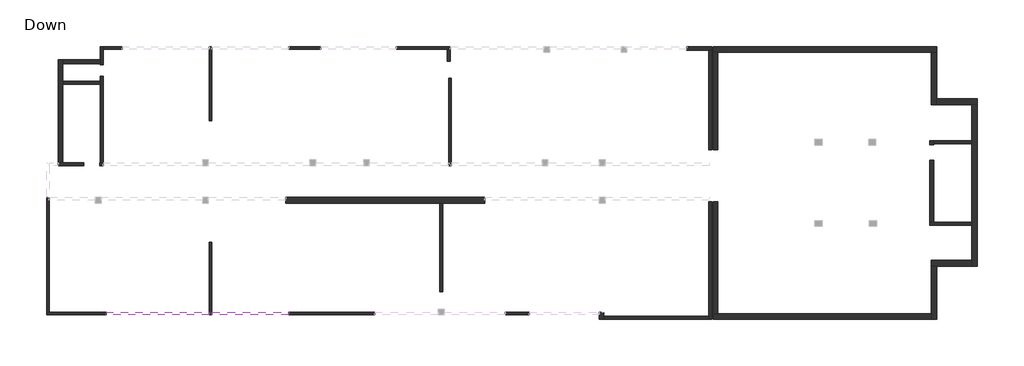
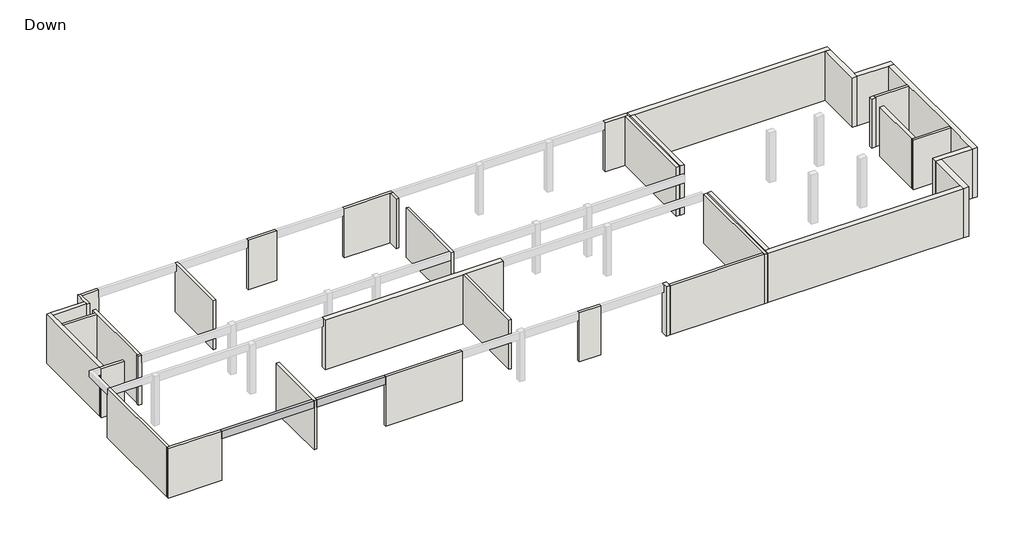
# One storey, part 1 of 2: 38 walls, 2 beams.
"""IFC4 building model written with IfcOpenShell, lengths in millimetres."""

from ifc_helpers import new_model, si_unit, origin, origin_with_axes, place, context, project, spatial, polyline, outline, extrude, faceted_brep, element, save

model = new_model("IFC4")

# Units and contexts
model_context = context("Model", 3, world=origin())
ifc_project = project(units=[si_unit("LENGTHUNIT", "METRE", prefix="MILLI")], contexts=[model_context])

# Site, building, storey
site = spatial("IfcSite", under=ifc_project)
building = spatial("IfcBuilding", under=site)
storey = spatial("IfcBuildingStorey", under=building, Name="Down", Elevation=0.0)

# Beams
placement = place(None, origin())
element("IfcBeam", 1, ObjectType="Concrete Rectengular Beam : 20/65", at=placement, inside=storey, context=model_context, shape_type="Brep", body=[
    faceted_brep([(-12691.9389092, -4274.5314528, 4000.0), (-12691.9389092, -4074.5314528, 4000.0), (-19792.231636, -4074.5314528, 4000.0), (-19792.231636, -4274.5314528, 4000.0), (-12691.9389092, -4274.5314528, 3400.0), (-19792.231636, -4274.5314528, 3400.0), (-12691.9389092, -4074.5314528, 3400.0), (-19792.231636, -4074.5314528, 3400.0), (-19792.231636, -4074.5314528, 3730.0), (-12691.9389092, -4074.5314528, 3730.0)], [[[0, 1, 2, 3]], [[4, 0, 3, 5]], [[6, 4, 5, 7]], [[6, 7, 8, 2, 1, 9]], [[0, 4, 6, 9, 1]], [[5, 3, 2, 8, 7]]]),
])
element("IfcBeam", 2, ObjectType="Concrete Rectengular Beam : 20/65", at=placement, inside=storey, context=model_context, shape_type="Brep", body=[
    faceted_brep([(-12491.9389092, -4074.5314528, 4000.0), (-12491.9389092, -4274.5314528, 4000.0), (-7191.8713568, -4274.5314528, 4000.0), (-7191.8713568, -4074.5314528, 4000.0), (-12491.9389092, -4274.5314528, 3400.0), (-7191.8713568, -4274.5314528, 3400.0), (-12491.9389092, -4074.5314528, 3400.0), (-7191.8713568, -4074.5314528, 3400.0), (-12491.9389092, -4074.5314528, 3730.0), (-7191.8713568, -4074.5314528, 3730.0)], [[[0, 1, 2, 3]], [[1, 4, 5, 2]], [[4, 6, 7, 5]], [[7, 6, 8, 0, 3, 9]], [[4, 1, 0, 8, 6]], [[2, 5, 7, 9, 3]]]),
])

# Walls
element("IfcWall", 3, ObjectType="20", at=placement, inside=storey, context=model_context, shape_type="Brep", body=[
    faceted_brep([(-19792.231636, -4074.5314528, 0.0), (-23692.1640837, -4074.5314528, 0.0), (-23892.1640837, -4074.5314528, 0.0), (-23892.1640837, -4074.5314528, 4000.0), (-23692.1640837, -4074.5314528, 4000.0), (-19792.231636, -4074.5314528, 4000.0), (-19792.231636, -4074.5314528, 3400.0), (-19792.231636, -4274.5314528, 0.0), (-19792.231636, -4274.5314528, 3400.0), (-19792.231636, -4274.5314528, 4000.0), (-23892.1640837, -4274.5314528, 4000.0), (-23892.1640837, -4274.5314528, 0.0)], [[[0, 1, 2, 3, 4, 5, 6]], [[7, 8, 9, 10, 11]], [[2, 1, 0, 7, 11]], [[5, 4, 3, 10, 9]], [[0, 6, 5, 9, 8, 7]], [[3, 2, 11, 10]]]),
])
element("IfcWall", 4, ObjectType="20", at=placement, inside=storey, context=model_context, shape_type="Brep", body=[
    faceted_brep([(-23692.1640837, -4074.5314528, 0.0), (-23692.1640837, 3825.8513439, 0.0), (-23692.1640837, 3825.8513439, 3500.0), (-23692.1640837, 3825.8513439, 4000.0), (-23692.1640837, 3625.8513439, 4000.0), (-23692.1640837, -4074.5314528, 4000.0), (-23692.1640837, -4074.5314528, 3730.0), (-23892.1640837, -4074.5314528, 0.0), (-23892.1640837, -4074.5314528, 4000.0), (-23892.1640837, 3825.8513439, 4000.0), (-23892.1640837, 3825.8513439, 3500.0), (-23892.1640837, 3825.8513439, 0.0)], [[[0, 1, 2, 3, 4, 5, 6]], [[7, 8, 9, 10, 11]], [[1, 0, 7, 11]], [[3, 2, 1, 11, 10, 9]], [[5, 4, 3, 9, 8]], [[0, 6, 5, 8, 7]]]),
])
element("IfcWall", 5, ObjectType="20", at=placement, inside=storey, context=model_context, shape_type="Brep", body=[
    faceted_brep([(-23092.0740139, 6025.0407157, 0.0), (-21341.6124061, 6025.0407157, 0.0), (-21341.6124061, 6025.0407157, 4000.0), (-23092.0740139, 6025.0407157, 4000.0), (-23092.0740139, 6025.0407157, 3500.0), (-23092.0740139, 6225.0407157, 0.0), (-23092.0740139, 6225.0407157, 3500.0), (-23092.0740139, 6225.0407157, 4000.0), (-22792.0740139, 6225.0407157, 4000.0), (-21341.6124061, 6225.0407157, 4000.0), (-21341.6124061, 6225.0407157, 0.0), (-22792.0740139, 6225.0407157, 0.0)], [[[0, 1, 2, 3, 4]], [[5, 6, 7, 8, 9, 10, 11]], [[1, 0, 5, 11, 10]], [[2, 1, 10, 9]], [[3, 2, 9, 8, 7]], [[0, 4, 3, 7, 6, 5]]]),
])
element("IfcWall", 6, ObjectType="20", at=placement, inside=storey, context=model_context, shape_type="Brep", body=[
    faceted_brep([(-20240.9594, 6025.0407157, 0.0), (-19991.1958333, 6025.0407157, 0.0), (-19991.1958333, 6025.0407157, 3400.0), (-19991.1958333, 6025.0407157, 4000.0), (-20240.9594, 6025.0407157, 4000.0), (-20240.9594, 6225.0407157, 0.0), (-20240.9594, 6225.0407157, 4000.0), (-20191.1958333, 6225.0407157, 4000.0), (-19991.1958333, 6225.0407157, 4000.0), (-19991.1958333, 6225.0407157, 3400.0), (-19991.1958333, 6225.0407157, 0.0), (-20191.1958333, 6225.0407157, 0.0)], [[[0, 1, 2, 3, 4]], [[5, 6, 7, 8, 9, 10, 11]], [[1, 0, 5, 11, 10]], [[4, 3, 8, 7, 6]], [[0, 4, 6, 5]], [[3, 2, 1, 10, 9, 8]]]),
])
element("IfcWall", 7, ObjectType="20", at=placement, inside=storey, context=model_context, shape_type="Brep", body=[
    faceted_brep([(-19991.1958333, 6225.0407157, 0.0), (-19991.1958333, 12173.8810669, 0.0), (-19991.1958333, 12173.8810669, 4000.0), (-19991.1958333, 6225.0407157, 4000.0), (-19991.1958333, 6225.0407157, 3730.0), (-20191.1958333, 6225.0407157, 0.0), (-20191.1958333, 6225.0407157, 4000.0), (-20191.1958333, 12173.8810669, 4000.0), (-20191.1958333, 12173.8810669, 0.0)], [[[0, 1, 2, 3, 4]], [[5, 6, 7, 8]], [[1, 0, 5, 8]], [[2, 1, 8, 7]], [[3, 2, 7, 6]], [[0, 4, 3, 6, 5]]]),
])
element("IfcWall", 8, ObjectType="20", at=placement, inside=storey, context=model_context, shape_type="SweptSolid", body=[
    extrude(outline(polyline([(-22792.0740139, 11825.6712043), (-20192.2766709, 11825.6712043), (-20192.2766709, 11625.6712043), (-22792.0740139, 11625.6712043), (-22792.0740139, 11825.6712043)])), origin_with_axes(), (0.0, 0.0, 1.0), 4000.0),
])
element("IfcWall", 9, ObjectType="20", at=placement, inside=storey, context=model_context, shape_type="Brep", body=[
    faceted_brep([(-19991.1958333, 12973.9711367, 0.0), (-19991.1958333, 14024.905611, 0.0), (-19991.1958333, 14224.905611, 0.0), (-19991.1958333, 14224.905611, 4000.0), (-19991.1958333, 14024.905611, 4000.0), (-19991.1958333, 12973.9711367, 4000.0), (-20191.1958333, 12973.9711367, 0.0), (-20191.1958333, 12973.9711367, 4000.0), (-20191.1958333, 13025.3334425, 4000.0), (-20191.1958333, 13325.3334425, 4000.0), (-20191.1958333, 14224.905611, 4000.0), (-20191.1958333, 14224.905611, 0.0), (-20191.1958333, 13325.3334425, 0.0), (-20191.1958333, 13025.3334425, 0.0)], [[[0, 1, 2, 3, 4, 5]], [[6, 7, 8, 9, 10, 11, 12, 13]], [[2, 1, 0, 6, 13, 12, 11]], [[5, 4, 3, 10, 9, 8, 7]], [[0, 5, 7, 6]], [[3, 2, 11, 10]]]),
])
element("IfcWall", 10, ObjectType="20", at=placement, inside=storey, context=model_context, shape_type="Brep", body=[
    faceted_brep([(-19991.1958333, 14024.905611, 0.0), (-18691.5786299, 14024.905611, 0.0), (-18691.5786299, 14024.905611, 3400.0), (-18691.5786299, 14024.905611, 4000.0), (-19991.1958333, 14024.905611, 4000.0), (-19991.1958333, 14024.905611, 3730.0), (-19991.1958333, 14224.905611, 0.0), (-19991.1958333, 14224.905611, 4000.0), (-18691.5786299, 14224.905611, 4000.0), (-18691.5786299, 14224.905611, 3400.0), (-18691.5786299, 14224.905611, 0.0)], [[[0, 1, 2, 3, 4, 5]], [[6, 7, 8, 9, 10]], [[1, 0, 6, 10]], [[3, 2, 1, 10, 9, 8]], [[4, 3, 8, 7]], [[0, 5, 4, 7, 6]]]),
])
element("IfcWall", 11, ObjectType="20", at=placement, inside=storey, context=model_context, shape_type="Brep", body=[
    faceted_brep([(-12690.9031064, 14224.905611, 0.0), (-12690.9031064, 9123.8022559, 0.0), (-12690.9031064, 9123.8022559, 3730.0), (-12690.9031064, 9123.8022559, 4000.0), (-12690.9031064, 14024.905611, 4000.0), (-12690.9031064, 14224.905611, 4000.0), (-12490.9031064, 14224.905611, 0.0), (-12490.9031064, 14224.905611, 4000.0), (-12490.9031064, 14024.905611, 4000.0), (-12490.9031064, 9123.8022559, 4000.0), (-12490.9031064, 9123.8022559, 3730.0), (-12490.9031064, 9123.8022559, 0.0)], [[[0, 1, 2, 3, 4, 5]], [[6, 7, 8, 9, 10, 11]], [[1, 0, 6, 11]], [[3, 2, 1, 11, 10, 9]], [[5, 4, 3, 9, 8, 7]], [[0, 5, 7, 6]]]),
])
element("IfcWall", 12, ObjectType="20", at=placement, inside=storey, context=model_context, shape_type="Brep", body=[
    faceted_brep([(-7191.8713568, 14024.905611, 0.0), (-4990.5653446, 14024.905611, 0.0), (-4990.5653446, 14024.905611, 3400.0), (-4990.5653446, 14024.905611, 4000.0), (-7191.8713568, 14024.905611, 4000.0), (-7191.8713568, 14024.905611, 3400.0), (-7191.8713568, 14224.905611, 0.0), (-7191.8713568, 14224.905611, 3400.0), (-7191.8713568, 14224.905611, 4000.0), (-4990.5653446, 14224.905611, 4000.0), (-4990.5653446, 14224.905611, 3400.0), (-4990.5653446, 14224.905611, 0.0)], [[[0, 1, 2, 3, 4, 5]], [[6, 7, 8, 9, 10, 11]], [[1, 0, 6, 11]], [[3, 2, 1, 11, 10, 9]], [[4, 3, 9, 8]], [[0, 5, 4, 8, 7, 6]]]),
])
element("IfcWall", 13, ObjectType="20", at=placement, inside=storey, context=model_context, shape_type="Brep", body=[
    faceted_brep([(207.9034687, 14024.905611, 0.0), (3733.1905662, 14024.905611, 0.0), (3933.1905662, 14024.905611, 0.0), (3933.1905662, 14024.905611, 3400.0), (3933.1905662, 14024.905611, 4000.0), (3733.1905662, 14024.905611, 4000.0), (207.9034687, 14024.905611, 4000.0), (207.9034687, 14024.905611, 3400.0), (207.9034687, 14224.905611, 0.0), (207.9034687, 14224.905611, 3400.0), (207.9034687, 14224.905611, 4000.0), (3933.1905662, 14224.905611, 4000.0), (3933.1905662, 14224.905611, 3400.0), (3933.1905662, 14224.905611, 0.0)], [[[0, 1, 2, 3, 4, 5, 6, 7]], [[8, 9, 10, 11, 12, 13]], [[2, 1, 0, 8, 13]], [[6, 5, 4, 11, 10]], [[0, 7, 6, 10, 9, 8]], [[4, 3, 2, 13, 12, 11]]]),
])
element("IfcWall", 14, ObjectType="20", at=placement, inside=storey, context=model_context, shape_type="Brep", body=[
    faceted_brep([(3733.1905662, 14024.905611, 0.0), (3733.1905662, 13223.7347035, 0.0), (3733.1905662, 13223.7347035, 3730.0), (3733.1905662, 13223.7347035, 4000.0), (3733.1905662, 14024.905611, 4000.0), (3733.1905662, 14024.905611, 3730.0), (3933.1905662, 14024.905611, 0.0), (3933.1905662, 14024.905611, 3730.0), (3933.1905662, 14024.905611, 4000.0), (3933.1905662, 13223.7347035, 4000.0), (3933.1905662, 13223.7347035, 3730.0), (3933.1905662, 13223.7347035, 0.0)], [[[0, 1, 2, 3, 4, 5]], [[6, 7, 8, 9, 10, 11]], [[1, 0, 6, 11]], [[3, 2, 1, 11, 10, 9]], [[4, 3, 9, 8]], [[0, 5, 4, 8, 7, 6]]]),
])
element("IfcWall", 15, ObjectType="20", at=placement, inside=storey, context=model_context, shape_type="Brep", body=[
    faceted_brep([(3809.3896205, 12023.5995988, 0.0), (3809.3896205, 6025.0407157, 0.0), (3809.3896205, 6025.0407157, 4000.0), (3809.3896205, 6225.0407157, 4000.0), (3809.3896205, 12023.5995988, 4000.0), (3809.3896205, 12023.5995988, 3730.0), (4009.3896205, 12023.5995988, 0.0), (4009.3896205, 12023.5995988, 3730.0), (4009.3896205, 12023.5995988, 4000.0), (4009.3896205, 6225.0407157, 4000.0), (4009.3896205, 6025.0407157, 4000.0), (4009.3896205, 6025.0407157, 0.0)], [[[0, 1, 2, 3, 4, 5]], [[6, 7, 8, 9, 10, 11]], [[1, 0, 6, 11]], [[2, 1, 11, 10]], [[4, 3, 2, 10, 9, 8]], [[0, 5, 4, 8, 7, 6]]]),
])
element("IfcWall", 16, ObjectType="20", at=placement, inside=storey, context=model_context, shape_type="Brep", body=[
    faceted_brep([(21760.6168215, 13975.1420442, 0.0), (21760.6168215, 7129.9270025, 0.0), (21760.6168215, 7129.9270025, 3730.0), (21760.6168215, 7129.9270025, 4000.0), (21760.6168215, 13975.1420442, 4000.0), (21760.6168215, 13975.1420442, 3730.0), (21960.6168215, 13975.1420442, 0.0), (21960.6168215, 13975.1420442, 4000.0), (21960.6168215, 7129.9270025, 4000.0), (21960.6168215, 7129.9270025, 0.0)], [[[0, 1, 2, 3, 4, 5]], [[6, 7, 8, 9]], [[1, 0, 6, 9]], [[3, 2, 1, 9, 8]], [[4, 3, 8, 7]], [[0, 5, 4, 7, 6]]]),
])
element("IfcWall", 17, ObjectType="20", at=placement, inside=storey, context=model_context, shape_type="Brep", body=[
    faceted_brep([(21760.6168215, 3525.2884076, 0.0), (21760.6168215, -4375.094389, 0.0), (21760.6168215, -4575.094389, 0.0), (21760.6168215, -4575.094389, 4000.0), (21760.6168215, -4375.094389, 4000.0), (21760.6168215, 3525.2884076, 4000.0), (21760.6168215, 3525.2884076, 3730.0), (21960.6168215, 3525.2884076, 0.0), (21960.6168215, 3525.2884076, 3730.0), (21960.6168215, 3525.2884076, 4000.0), (21960.6168215, 3516.821846, 4000.0), (21960.6168215, -4575.094389, 4000.0), (21960.6168215, -4575.094389, 0.0)], [[[0, 1, 2, 3, 4, 5, 6]], [[7, 8, 9, 10, 11, 12]], [[2, 1, 0, 7, 12]], [[5, 4, 3, 11, 10, 9]], [[0, 6, 5, 9, 8, 7]], [[3, 2, 12, 11]]]),
])
element("IfcWall", 18, ObjectType="20", at=placement, inside=storey, context=model_context, shape_type="Brep", body=[
    faceted_brep([(21760.6168215, -4375.094389, 0.0), (14509.4796903, -4375.094389, 0.0), (14509.4796903, -4375.094389, 3730.0), (14509.4796903, -4375.094389, 4000.0), (21760.6168215, -4375.094389, 4000.0), (21760.6168215, -4375.094389, 3730.0), (21760.6168215, -4575.094389, 0.0), (21760.6168215, -4575.094389, 4000.0), (14509.4796903, -4575.094389, 4000.0), (14509.4796903, -4575.094389, 0.0)], [[[0, 1, 2, 3, 4, 5]], [[6, 7, 8, 9]], [[1, 0, 6, 9]], [[4, 3, 8, 7]], [[0, 5, 4, 7, 6]], [[3, 2, 1, 9, 8]]]),
])
element("IfcWall", 19, ObjectType="20", at=placement, inside=storey, context=model_context, shape_type="Brep", body=[
    faceted_brep([(9358.1399019, -4074.5314528, 0.0), (7709.2770332, -4074.5314528, 0.0), (7709.2770332, -4074.5314528, 3400.0), (7709.2770332, -4074.5314528, 4000.0), (9358.1399019, -4074.5314528, 4000.0), (9358.1399019, -4074.5314528, 3400.0), (9358.1399019, -4274.5314528, 0.0), (9358.1399019, -4274.5314528, 3400.0), (9358.1399019, -4274.5314528, 4000.0), (7709.2770332, -4274.5314528, 4000.0), (7709.2770332, -4274.5314528, 3400.0), (7709.2770332, -4274.5314528, 0.0)], [[[0, 1, 2, 3, 4, 5]], [[6, 7, 8, 9, 10, 11]], [[1, 0, 6, 11]], [[3, 2, 1, 11, 10, 9]], [[4, 3, 9, 8]], [[0, 5, 4, 8, 7, 6]]]),
])
element("IfcWall", 20, ObjectType="20", at=placement, inside=storey, context=model_context, shape_type="Brep", body=[
    faceted_brep([(-1290.6779319, -4074.5314528, 0.0), (-7191.8713568, -4074.5314528, 0.0), (-7191.8713568, -4074.5314528, 3400.0), (-7191.8713568, -4074.5314528, 4000.0), (-1290.6779319, -4074.5314528, 4000.0), (-1290.6779319, -4074.5314528, 3400.0), (-1290.6779319, -4274.5314528, 0.0), (-1290.6779319, -4274.5314528, 3400.0), (-1290.6779319, -4274.5314528, 4000.0), (-7191.8713568, -4274.5314528, 4000.0), (-7191.8713568, -4274.5314528, 3400.0), (-7191.8713568, -4274.5314528, 0.0)], [[[0, 1, 2, 3, 4, 5]], [[6, 7, 8, 9, 10, 11]], [[1, 0, 6, 11]], [[3, 2, 1, 11, 10, 9]], [[4, 3, 9, 8]], [[0, 5, 4, 8, 7, 6]]]),
])
element("IfcWall", 21, ObjectType="20", at=placement, inside=storey, context=model_context, shape_type="Brep", body=[
    faceted_brep([(-12691.9389092, 724.9731633, 0.0), (-12691.9389092, -4274.5314528, 0.0), (-12691.9389092, -4274.5314528, 4000.0), (-12691.9389092, -4074.5314528, 4000.0), (-12691.9389092, 724.9731633, 4000.0), (-12691.9389092, 724.9731633, 3730.0), (-12491.9389092, 724.9731633, 0.0), (-12491.9389092, 724.9731633, 3730.0), (-12491.9389092, 724.9731633, 4000.0), (-12491.9389092, -4074.5314528, 4000.0), (-12491.9389092, -4274.5314528, 4000.0), (-12491.9389092, -4274.5314528, 0.0)], [[[0, 1, 2, 3, 4, 5]], [[6, 7, 8, 9, 10, 11]], [[1, 0, 6, 11]], [[2, 1, 11, 10]], [[4, 3, 2, 10, 9, 8]], [[0, 5, 4, 8, 7, 6]]]),
])
element("IfcWall", 22, ObjectType="20", at=placement, inside=storey, context=model_context, shape_type="Brep", body=[
    faceted_brep([(3409.2995507, -2674.3513132, 0.0), (3409.2995507, 3425.806309, 0.0), (3409.2995507, 3425.806309, 3730.0), (3409.2995507, 3425.806309, 4000.0), (3409.2995507, -2674.3513132, 4000.0), (3409.2995507, -2674.3513132, 3730.0), (3209.2995507, -2674.3513132, 0.0), (3209.2995507, -2674.3513132, 3730.0), (3209.2995507, -2674.3513132, 4000.0), (3209.2995507, 3425.806309, 4000.0), (3209.2995507, 3425.806309, 3730.0), (3209.2995507, 3425.806309, 0.0)], [[[0, 1, 2, 3, 4, 5]], [[6, 7, 8, 9, 10, 11]], [[1, 0, 6, 11]], [[4, 3, 9, 8]], [[0, 5, 4, 8, 7, 6]], [[3, 2, 1, 11, 10, 9]]]),
])
element("IfcWall", 23, ObjectType="20", at=placement, inside=storey, context=model_context, shape_type="Brep", body=[
    faceted_brep([(39861.089688, 2122.9916276, 0.0), (37261.2473102, 2122.9916276, 0.0), (36961.2473102, 2122.9916276, 0.0), (36961.2473102, 2122.9916276, 4000.0), (37261.2473102, 2122.9916276, 4000.0), (39861.089688, 2122.9916276, 4000.0), (39861.089688, 1922.9916276, 0.0), (39861.089688, 1922.9916276, 3730.0), (39861.089688, 1922.9916276, 4000.0), (36961.2473102, 1922.9916276, 4000.0), (36961.2473102, 1922.9916276, 3730.0), (36961.2473102, 1922.9916276, 0.0)], [[[0, 1, 2, 3, 4, 5]], [[6, 7, 8, 9, 10, 11]], [[2, 1, 0, 6, 11]], [[5, 4, 3, 9, 8]], [[0, 5, 8, 7, 6]], [[3, 2, 11, 10, 9]]]),
])
element("IfcWall", 24, ObjectType="20", at=placement, inside=storey, context=model_context, shape_type="Brep", body=[
    faceted_brep([(39861.089688, 7724.7029539, 0.0), (37261.2473102, 7724.7029539, 0.0), (37261.2473102, 7724.7029539, 4000.0), (39861.089688, 7724.7029539, 4000.0), (39861.089688, 7724.7029539, 3730.0), (39861.089688, 7524.7029539, 0.0), (39861.089688, 7524.7029539, 3730.0), (39861.089688, 7524.7029539, 4000.0), (37261.2473102, 7524.7029539, 4000.0), (37261.2473102, 7524.7029539, 3730.0), (37261.2473102, 7524.7029539, 0.0)], [[[0, 1, 2, 3, 4]], [[5, 6, 7, 8, 9, 10]], [[1, 0, 5, 10]], [[3, 2, 8, 7]], [[0, 4, 3, 7, 6, 5]], [[2, 1, 10, 9, 8]]]),
])
element("IfcWall", 25, ObjectType="25", at=placement, inside=storey, context=model_context, shape_type="Brep", body=[
    faceted_brep([(20235.5548985, 13975.1420442, 0.0), (21760.6168215, 13975.1420442, 0.0), (21960.6168215, 13975.1420442, 0.0), (21960.6168215, 13975.1420442, 4000.0), (21760.6168215, 13975.1420442, 4000.0), (20235.5548985, 13975.1420442, 4000.0), (20235.5548985, 13975.1420442, 3730.0), (20235.5548985, 14225.1420442, 0.0), (20235.5548985, 14225.1420442, 3400.0), (20235.5548985, 14225.1420442, 4000.0), (21960.6168215, 14225.1420442, 4000.0), (21960.6168215, 14225.1420442, 0.0), (20235.5548985, 14025.1420442, 4000.0)], [[[0, 1, 2, 3, 4, 5, 6]], [[7, 8, 9, 10, 11]], [[2, 1, 0, 7, 11]], [[5, 4, 3, 10, 9, 12]], [[0, 6, 5, 12, 9, 8, 7]], [[3, 2, 11, 10]]]),
])
element("IfcWall", 26, ObjectType="30", at=placement, inside=storey, context=model_context, shape_type="Brep", body=[
    faceted_brep([(-22792.0740139, 6225.0407157, 0.0), (-22792.0740139, 11625.6712043, 0.0), (-22792.0740139, 11825.6712043, 0.0), (-22792.0740139, 13025.3334425, 0.0), (-22792.0740139, 13325.3334425, 0.0), (-22792.0740139, 13325.3334425, 4000.0), (-22792.0740139, 13025.3334425, 4000.0), (-22792.0740139, 11825.6712043, 4000.0), (-22792.0740139, 11625.6712043, 4000.0), (-22792.0740139, 6225.0407157, 4000.0), (-23092.0740139, 6225.0407157, 0.0), (-23092.0740139, 6225.0407157, 4000.0), (-23092.0740139, 13325.3334425, 4000.0), (-23092.0740139, 13325.3334425, 0.0)], [[[0, 1, 2, 3, 4, 5, 6, 7, 8, 9]], [[10, 11, 12, 13]], [[4, 3, 2, 1, 0, 10, 13]], [[9, 8, 7, 6, 5, 12, 11]], [[0, 9, 11, 10]], [[5, 4, 13, 12]]]),
])
element("IfcWall", 27, ObjectType="30", at=placement, inside=storey, context=model_context, shape_type="SweptSolid", body=[
    extrude(outline(polyline([(-20191.1958333, 13025.3334425), (-22792.0740139, 13025.3334425), (-22792.0740139, 13325.3334425), (-20191.1958333, 13325.3334425), (-20191.1958333, 13025.3334425)])), origin_with_axes(), (0.0, 0.0, 1.0), 4000.0),
])
element("IfcWall", 28, ObjectType="30", at=placement, inside=storey, context=model_context, shape_type="Brep", body=[
    faceted_brep([(14509.4796903, -4575.094389, 0.0), (14509.4796903, -4375.094389, 0.0), (14509.4796903, -4075.5672555, 0.0), (14509.4796903, -4075.5672555, 4000.0), (14509.4796903, -4375.094389, 4000.0), (14509.4796903, -4575.094389, 4000.0), (14209.4796903, -4575.094389, 0.0), (14209.4796903, -4575.094389, 4000.0), (14209.4796903, -4075.5672555, 4000.0), (14209.4796903, -4075.5672555, 0.0)], [[[0, 1, 2, 3, 4, 5]], [[6, 7, 8, 9]], [[2, 1, 0, 6, 9]], [[3, 2, 9, 8]], [[5, 4, 3, 8, 7]], [[0, 5, 7, 6]]]),
])
element("IfcWall", 29, ObjectType="30", at=placement, inside=storey, context=model_context, shape_type="Brep", body=[
    faceted_brep([(22060.0989202, 13824.905611, 0.0), (22060.0989202, 7129.9270025, 0.0), (22060.0989202, 7129.9270025, 4000.0), (22060.0989202, 13824.905611, 4000.0), (22360.0989202, 13824.905611, 0.0), (22360.0989202, 13824.905611, 3730.0), (22360.0989202, 13824.905611, 4000.0), (22360.0989202, 7129.9270025, 4000.0), (22360.0989202, 7129.9270025, 3730.0), (22360.0989202, 7129.9270025, 0.0)], [[[0, 1, 2, 3]], [[4, 5, 6, 7, 8, 9]], [[1, 0, 4, 9]], [[2, 1, 9, 8, 7]], [[3, 2, 7, 6]], [[0, 3, 6, 5, 4]]]),
])
element("IfcWall", 30, ObjectType="30", at=placement, inside=storey, context=model_context, shape_type="Brep", body=[
    faceted_brep([(22060.0989202, 3516.821846, 0.0), (22060.0989202, -4175.094389, 0.0), (22060.0989202, -4175.094389, 4000.0), (22060.0989202, 3516.821846, 4000.0), (22360.0989202, 3516.821846, 0.0), (22360.0989202, 3516.821846, 3730.0), (22360.0989202, 3516.821846, 4000.0), (22360.0989202, -4175.094389, 4000.0), (22360.0989202, -4175.094389, 0.0)], [[[0, 1, 2, 3]], [[4, 5, 6, 7, 8]], [[1, 0, 4, 8]], [[3, 2, 7, 6]], [[0, 3, 6, 5, 4]], [[2, 1, 8, 7]]]),
])
element("IfcWall", 31, ObjectType="30", at=placement, inside=storey, context=model_context, shape_type="Brep", body=[
    faceted_brep([(36961.2473102, 7724.7029539, 0.0), (36961.2473102, 7474.9393871, 0.0), (36961.2473102, 7474.9393871, 3730.0), (36961.2473102, 7474.9393871, 4000.0), (36961.2473102, 7724.7029539, 4000.0), (36961.2473102, 7724.7029539, 3730.0), (37261.2473102, 7724.7029539, 0.0), (37261.2473102, 7724.7029539, 4000.0), (37261.2473102, 7524.7029539, 4000.0), (37261.2473102, 7474.9393871, 4000.0), (37261.2473102, 7474.9393871, 3730.0), (37261.2473102, 7474.9393871, 0.0), (37261.2473102, 7524.7029539, 0.0)], [[[0, 1, 2, 3, 4, 5]], [[6, 7, 8, 9, 10, 11, 12]], [[1, 0, 6, 12, 11]], [[3, 2, 1, 11, 10, 9]], [[4, 3, 9, 8, 7]], [[0, 5, 4, 7, 6]]]),
])
element("IfcWall", 32, ObjectType="30", at=placement, inside=storey, context=model_context, shape_type="Brep", body=[
    faceted_brep([(36961.2473102, 6374.286381, 0.0), (36961.2473102, 2122.9916276, 0.0), (36961.2473102, 2122.9916276, 4000.0), (36961.2473102, 6374.286381, 4000.0), (36961.2473102, 6374.286381, 3730.0), (37261.2473102, 6374.286381, 0.0), (37261.2473102, 6374.286381, 4000.0), (37261.2473102, 2122.9916276, 4000.0), (37261.2473102, 2122.9916276, 0.0)], [[[0, 1, 2, 3, 4]], [[5, 6, 7, 8]], [[1, 0, 5, 8]], [[3, 2, 7, 6]], [[0, 4, 3, 6, 5]], [[2, 1, 8, 7]]]),
])
element("IfcWall", 33, ObjectType="40", at=placement, inside=storey, context=model_context, shape_type="Brep", body=[
    faceted_brep([(-7390.8355541, 3425.806309, 0.0), (3209.2995507, 3425.806309, 0.0), (3409.2995507, 3425.806309, 0.0), (6309.1644459, 3425.806309, 0.0), (6309.1644459, 3425.806309, 3730.0), (6309.1644459, 3425.806309, 4000.0), (3409.2995507, 3425.806309, 4000.0), (3209.2995507, 3425.806309, 4000.0), (-7390.8355541, 3425.806309, 4000.0), (-7390.8355541, 3425.806309, 3730.0), (-7390.8355541, 3825.806309, 0.0), (-7390.8355541, 3825.806309, 4000.0), (6309.1644459, 3825.806309, 4000.0), (6309.1644459, 3825.806309, 0.0), (6309.1644459, 3625.8513439, 4000.0), (-7390.8355541, 3625.8513439, 4000.0)], [[[0, 1, 2, 3, 4, 5, 6, 7, 8, 9]], [[10, 11, 12, 13]], [[3, 2, 1, 0, 10, 13]], [[5, 4, 3, 13, 12, 14]], [[8, 7, 6, 5, 14, 12, 11, 15]], [[0, 9, 8, 15, 11, 10]]]),
])
element("IfcWall", 34, ObjectType="40", at=placement, inside=storey, context=model_context, shape_type="Brep", body=[
    faceted_brep([(22060.0989202, 13824.905611, 0.0), (22360.0989202, 13824.905611, 0.0), (37060.7744437, 13824.905611, 0.0), (37460.7744437, 13824.905611, 0.0), (37460.7744437, 13824.905611, 4000.0), (37060.7744437, 13824.905611, 4000.0), (22360.0989202, 13824.905611, 4000.0), (22060.0989202, 13824.905611, 4000.0), (22060.0989202, 14224.905611, 0.0), (22060.0989202, 14224.905611, 4000.0), (37460.7744437, 14224.905611, 4000.0), (37460.7744437, 14224.905611, 0.0)], [[[0, 1, 2, 3, 4, 5, 6, 7]], [[8, 9, 10, 11]], [[3, 2, 1, 0, 8, 11]], [[7, 6, 5, 4, 10, 9]], [[4, 3, 11, 10]], [[0, 7, 9, 8]]]),
])
element("IfcWall", 35, ObjectType="40", at=placement, inside=storey, context=model_context, shape_type="Brep", body=[
    faceted_brep([(37060.7744437, 13824.905611, 0.0), (37060.7744437, 10224.905611, 0.0), (37060.7744437, 10224.905611, 3730.0), (37060.7744437, 10224.905611, 4000.0), (37060.7744437, 13824.905611, 4000.0), (37060.7744437, 13824.905611, 3730.0), (37460.7744437, 13824.905611, 0.0), (37460.7744437, 13824.905611, 4000.0), (37460.7744437, 10624.905611, 4000.0), (37460.7744437, 10224.905611, 4000.0), (37460.7744437, 10224.905611, 0.0), (37460.7744437, 10624.905611, 0.0)], [[[0, 1, 2, 3, 4, 5]], [[6, 7, 8, 9, 10, 11]], [[1, 0, 6, 11, 10]], [[4, 3, 9, 8, 7]], [[0, 5, 4, 7, 6]], [[3, 2, 1, 10, 9]]]),
])
element("IfcWall", 36, ObjectType="40", at=placement, inside=storey, context=model_context, shape_type="Brep", body=[
    faceted_brep([(37460.7744437, 10224.905611, 0.0), (39861.089688, 10224.905611, 0.0), (40261.089688, 10224.905611, 0.0), (40261.089688, 10224.905611, 4000.0), (39861.089688, 10224.905611, 4000.0), (37460.7744437, 10224.905611, 4000.0), (37460.7744437, 10624.905611, 0.0), (37460.7744437, 10624.905611, 4000.0), (40261.089688, 10624.905611, 4000.0), (40261.089688, 10624.905611, 0.0)], [[[0, 1, 2, 3, 4, 5]], [[6, 7, 8, 9]], [[2, 1, 0, 6, 9]], [[5, 4, 3, 8, 7]], [[0, 5, 7, 6]], [[3, 2, 9, 8]]]),
])
element("IfcWall", 37, ObjectType="40", at=placement, inside=storey, context=model_context, shape_type="Brep", body=[
    faceted_brep([(39861.089688, 10224.905611, 0.0), (39861.089688, 7724.7029539, 0.0), (39861.089688, 7524.7029539, 0.0), (39861.089688, 2122.9916276, 0.0), (39861.089688, 1922.9916276, 0.0), (39861.089688, -500.6066611, 0.0), (39861.089688, -900.6066611, 0.0), (39861.089688, -900.6066611, 4000.0), (39861.089688, -500.6066611, 4000.0), (39861.089688, 1922.9916276, 4000.0), (39861.089688, 2122.9916276, 4000.0), (39861.089688, 6374.286381, 4000.0), (39861.089688, 7524.7029539, 4000.0), (39861.089688, 7724.7029539, 4000.0), (39861.089688, 10224.905611, 4000.0), (39861.089688, 10224.905611, 3730.0), (40261.089688, 10224.905611, 0.0), (40261.089688, 10224.905611, 4000.0), (40261.089688, -900.6066611, 4000.0), (40261.089688, -900.6066611, 0.0)], [[[0, 1, 2, 3, 4, 5, 6, 7, 8, 9, 10, 11, 12, 13, 14, 15]], [[16, 17, 18, 19]], [[6, 5, 4, 3, 2, 1, 0, 16, 19]], [[14, 13, 12, 11, 10, 9, 8, 7, 18, 17]], [[0, 15, 14, 17, 16]], [[7, 6, 19, 18]]]),
])
element("IfcWall", 38, ObjectType="40", at=placement, inside=storey, context=model_context, shape_type="Brep", body=[
    faceted_brep([(39861.089688, -500.6066611, 0.0), (37060.7294088, -500.6066611, 0.0), (37060.7294088, -500.6066611, 3730.0), (37060.7294088, -500.6066611, 4000.0), (39861.089688, -500.6066611, 4000.0), (39861.089688, -500.6066611, 3730.0), (39861.089688, -900.6066611, 0.0), (39861.089688, -900.6066611, 4000.0), (37460.7294088, -900.6066611, 4000.0), (37060.7294088, -900.6066611, 4000.0), (37060.7294088, -900.6066611, 0.0), (37460.7294088, -900.6066611, 0.0)], [[[0, 1, 2, 3, 4, 5]], [[6, 7, 8, 9, 10, 11]], [[1, 0, 6, 11, 10]], [[4, 3, 9, 8, 7]], [[0, 5, 4, 7, 6]], [[3, 2, 1, 10, 9]]]),
])
element("IfcWall", 39, ObjectType="40", at=placement, inside=storey, context=model_context, shape_type="Brep", body=[
    faceted_brep([(37060.7294088, -900.6066611, 0.0), (37060.7294088, -4175.094389, 0.0), (37060.7294088, -4575.094389, 0.0), (37060.7294088, -4575.094389, 4000.0), (37060.7294088, -4175.094389, 4000.0), (37060.7294088, -900.6066611, 4000.0), (37460.7294088, -900.6066611, 0.0), (37460.7294088, -900.6066611, 4000.0), (37460.7294088, -4575.094389, 4000.0), (37460.7294088, -4575.094389, 0.0)], [[[0, 1, 2, 3, 4, 5]], [[6, 7, 8, 9]], [[2, 1, 0, 6, 9]], [[5, 4, 3, 8, 7]], [[0, 5, 7, 6]], [[3, 2, 9, 8]]]),
])
element("IfcWall", 40, ObjectType="40", at=placement, inside=storey, context=model_context, shape_type="Brep", body=[
    faceted_brep([(37060.7294088, -4175.094389, 0.0), (22360.0989202, -4175.094389, 0.0), (22060.0989202, -4175.094389, 0.0), (22060.0989202, -4175.094389, 4000.0), (22360.0989202, -4175.094389, 4000.0), (37060.7294088, -4175.094389, 4000.0), (37060.7294088, -4175.094389, 3730.0), (37060.7294088, -4575.094389, 0.0), (37060.7294088, -4575.094389, 4000.0), (22060.0989202, -4575.094389, 4000.0), (22060.0989202, -4575.094389, 0.0)], [[[0, 1, 2, 3, 4, 5, 6]], [[7, 8, 9, 10]], [[2, 1, 0, 7, 10]], [[5, 4, 3, 9, 8]], [[0, 6, 5, 8, 7]], [[3, 2, 10, 9]]]),
])

save(model, "model.ifc")

# Revit data of these elements
# Project information
#   Project Issue Date = "Issue Date"
#   Project Status = "Project Status"
#   Client Name = "לקוח"
#   Project Address = "Enter address here"
#   Project Name = "Project 020"
#   Project Number = "מספר פרויקט"
# Type "Concrete Rectengular Beam : 20/65"
#   Length [instance default] = 152.4 cm
#   b = 20 cm
#   h = 60 cm
#   Structural Material [instance default] = Concrete
#   Assembly Code = ""
# Type "20"
#   Layers, outside or top first: 20 cm "Concrete" (function 1)
# Type "25"
#   Layers, outside or top first: 25 cm "Concrete" (function 1)
# Type "30"
#   Layers, outside or top first: 30 cm "Concrete" (function 1)
# Type "40"
#   Layers, outside or top first: 40 cm "Concrete" (function 1)
# Element 1 (IfcBeam, "Concrete Rectengular Beam : 20/65")
#   Comments = ""
#   Mark = "B15"
#   SOFiSTiK_AMG_Comments = ""
#   SOFiSTiK_AMG_Scheduled = yes
#   SOFiSTiK_AMG_Adjusted = yes
#   Structural Material = Concrete
#   Phase Created = New Construction
#   Materials on its faces: "Concrete"
# Element 2 (IfcBeam, "Concrete Rectengular Beam : 20/65")
#   Comments = ""
#   Mark = "B16"
#   SOFiSTiK_AMG_Comments = ""
#   SOFiSTiK_AMG_Scheduled = yes
#   SOFiSTiK_AMG_Adjusted = yes
#   Structural Material = Concrete
#   Phase Created = New Construction
#   Materials on its faces: "Concrete"
# Element 3 (IfcWall, "20")
#   Comments = ""
#   Mark = "W1"
#   SOFiSTiK_EdgeZones = "W1"
#   SOFiSTiK_AMG_Comments = ""
#   Top Offset = 0 cm
#   Base Offset = 0 cm
#   Unconnected Height = 400 cm
#   wall height = 400 cm
#   SOFiSTiK_AMG_Scheduled = yes
#   SOFiSTiK_AMG_Adjusted = yes
#   Phase Created = New Construction
#   Base Constraint = Down
#   Top Constraint = Typical Floor
#   Materials on its faces: "Concrete"
# Element 4 (IfcWall, "20")
#   Comments = ""
#   Mark = "W2"
#   SOFiSTiK_EdgeZones = "W2"
#   SOFiSTiK_AMG_Comments = ""
#   Top Offset = 0 cm
#   Base Offset = 0 cm
#   Unconnected Height = 400 cm
#   wall height = 400 cm
#   SOFiSTiK_AMG_Scheduled = yes
#   SOFiSTiK_AMG_Adjusted = yes
#   Phase Created = New Construction
#   Base Constraint = Down
#   Top Constraint = Typical Floor
#   Materials on its faces: "Concrete"
# Element 5 (IfcWall, "20")
#   Comments = ""
#   Mark = "W3"
#   SOFiSTiK_EdgeZones = "W3"
#   SOFiSTiK_AMG_Comments = ""
#   Top Offset = 0 cm
#   Base Offset = 0 cm
#   Unconnected Height = 400 cm
#   wall height = 400 cm
#   SOFiSTiK_AMG_Scheduled = yes
#   SOFiSTiK_AMG_Adjusted = yes
#   Phase Created = New Construction
#   Base Constraint = Down
#   Top Constraint = Typical Floor
#   Materials on its faces: "Concrete"
# Element 6 (IfcWall, "20")
#   Comments = ""
#   Mark = "W4"
#   SOFiSTiK_EdgeZones = "W4"
#   SOFiSTiK_AMG_Comments = ""
#   Top Offset = 0 cm
#   Base Offset = 0 cm
#   Unconnected Height = 400 cm
#   wall height = 400 cm
#   SOFiSTiK_AMG_Scheduled = yes
#   SOFiSTiK_AMG_Adjusted = yes
#   Phase Created = New Construction
#   Base Constraint = Down
#   Top Constraint = Typical Floor
#   Materials on its faces: "Concrete"
# Element 7 (IfcWall, "20")
#   Comments = ""
#   Mark = "W5"
#   SOFiSTiK_EdgeZones = "W5"
#   SOFiSTiK_AMG_Comments = ""
#   Top Offset = 0 cm
#   Base Offset = 0 cm
#   Unconnected Height = 400 cm
#   wall height = 400 cm
#   SOFiSTiK_AMG_Scheduled = yes
#   SOFiSTiK_AMG_Adjusted = yes
#   Phase Created = New Construction
#   Base Constraint = Down
#   Top Constraint = Typical Floor
#   Materials on its faces: "Concrete"
# Element 8 (IfcWall, "20")
#   Comments = ""
#   Mark = "W6"
#   SOFiSTiK_EdgeZones = "W6"
#   SOFiSTiK_AMG_Comments = ""
#   Top Offset = 0 cm
#   Base Offset = 0 cm
#   Unconnected Height = 400 cm
#   wall height = 400 cm
#   SOFiSTiK_AMG_Scheduled = yes
#   SOFiSTiK_AMG_Adjusted = yes
#   Phase Created = New Construction
#   Base Constraint = Down
#   Top Constraint = Typical Floor
#   Materials on its faces: "Concrete"
# Element 9 (IfcWall, "20")
#   Comments = ""
#   Mark = "W7"
#   SOFiSTiK_EdgeZones = "W7"
#   SOFiSTiK_AMG_Comments = ""
#   Top Offset = 0 cm
#   Base Offset = 0 cm
#   Unconnected Height = 400 cm
#   wall height = 400 cm
#   SOFiSTiK_AMG_Scheduled = yes
#   SOFiSTiK_AMG_Adjusted = yes
#   Phase Created = New Construction
#   Base Constraint = Down
#   Top Constraint = Typical Floor
#   Materials on its faces: "Concrete"
# Element 10 (IfcWall, "20")
#   Comments = ""
#   Mark = "W8"
#   SOFiSTiK_EdgeZones = "W8"
#   SOFiSTiK_AMG_Comments = ""
#   Top Offset = 0 cm
#   Base Offset = 0 cm
#   Unconnected Height = 400 cm
#   wall height = 400 cm
#   SOFiSTiK_AMG_Scheduled = yes
#   SOFiSTiK_AMG_Adjusted = yes
#   Phase Created = New Construction
#   Base Constraint = Down
#   Top Constraint = Typical Floor
#   Materials on its faces: "Concrete"
# Element 11 (IfcWall, "20")
#   Comments = ""
#   Mark = "W9"
#   SOFiSTiK_EdgeZones = "W9"
#   SOFiSTiK_AMG_Comments = ""
#   Top Offset = 0 cm
#   Base Offset = 0 cm
#   Unconnected Height = 400 cm
#   wall height = 400 cm
#   SOFiSTiK_AMG_Scheduled = yes
#   SOFiSTiK_AMG_Adjusted = yes
#   Phase Created = New Construction
#   Base Constraint = Down
#   Top Constraint = Typical Floor
#   Materials on its faces: "Concrete"
# Element 12 (IfcWall, "20")
#   Comments = ""
#   Mark = "W10"
#   SOFiSTiK_EdgeZones = "W10"
#   SOFiSTiK_AMG_Comments = ""
#   Top Offset = 0 cm
#   Base Offset = 0 cm
#   Unconnected Height = 400 cm
#   wall height = 400 cm
#   SOFiSTiK_AMG_Scheduled = yes
#   SOFiSTiK_AMG_Adjusted = yes
#   Phase Created = New Construction
#   Base Constraint = Down
#   Top Constraint = Typical Floor
#   Materials on its faces: "Concrete"
# Element 13 (IfcWall, "20")
#   Comments = ""
#   Mark = "W11"
#   SOFiSTiK_EdgeZones = "W11"
#   SOFiSTiK_AMG_Comments = ""
#   Top Offset = 0 cm
#   Base Offset = 0 cm
#   Unconnected Height = 400 cm
#   wall height = 400 cm
#   SOFiSTiK_AMG_Scheduled = yes
#   SOFiSTiK_AMG_Adjusted = yes
#   Phase Created = New Construction
#   Base Constraint = Down
#   Top Constraint = Typical Floor
#   Materials on its faces: "Concrete"
# Element 14 (IfcWall, "20")
#   Comments = ""
#   Mark = "W12"
#   SOFiSTiK_EdgeZones = "W12"
#   SOFiSTiK_AMG_Comments = ""
#   Top Offset = 0 cm
#   Base Offset = 0 cm
#   Unconnected Height = 400 cm
#   wall height = 400 cm
#   SOFiSTiK_AMG_Scheduled = yes
#   SOFiSTiK_AMG_Adjusted = yes
#   Phase Created = New Construction
#   Base Constraint = Down
#   Top Constraint = Typical Floor
#   Materials on its faces: "Concrete"
# Element 15 (IfcWall, "20")
#   Comments = ""
#   Mark = "W13"
#   SOFiSTiK_EdgeZones = "W13"
#   SOFiSTiK_AMG_Comments = ""
#   Top Offset = 0 cm
#   Base Offset = 0 cm
#   Unconnected Height = 400 cm
#   wall height = 400 cm
#   SOFiSTiK_AMG_Scheduled = yes
#   SOFiSTiK_AMG_Adjusted = yes
#   Phase Created = New Construction
#   Base Constraint = Down
#   Top Constraint = Typical Floor
#   Materials on its faces: "Concrete"
# Element 16 (IfcWall, "20")
#   Comments = ""
#   Mark = "W14"
#   SOFiSTiK_EdgeZones = "W14"
#   SOFiSTiK_AMG_Comments = ""
#   Top Offset = 0 cm
#   Base Offset = 0 cm
#   Unconnected Height = 400 cm
#   wall height = 400 cm
#   SOFiSTiK_AMG_Scheduled = yes
#   SOFiSTiK_AMG_Adjusted = yes
#   Phase Created = New Construction
#   Base Constraint = Down
#   Top Constraint = Typical Floor
#   Materials on its faces: "Concrete"
# Element 17 (IfcWall, "20")
#   Comments = ""
#   Mark = "W15"
#   SOFiSTiK_EdgeZones = "W15"
#   SOFiSTiK_AMG_Comments = ""
#   Top Offset = 0 cm
#   Base Offset = 0 cm
#   Unconnected Height = 400 cm
#   wall height = 400 cm
#   SOFiSTiK_AMG_Scheduled = yes
#   SOFiSTiK_AMG_Adjusted = yes
#   Phase Created = New Construction
#   Base Constraint = Down
#   Top Constraint = Typical Floor
#   Materials on its faces: "Concrete"
# Element 18 (IfcWall, "20")
#   Comments = ""
#   Mark = "W16"
#   SOFiSTiK_EdgeZones = "W16"
#   SOFiSTiK_AMG_Comments = ""
#   Top Offset = 0 cm
#   Base Offset = 0 cm
#   Unconnected Height = 400 cm
#   wall height = 400 cm
#   SOFiSTiK_AMG_Scheduled = yes
#   SOFiSTiK_AMG_Adjusted = yes
#   Phase Created = New Construction
#   Base Constraint = Down
#   Top Constraint = Typical Floor
#   Materials on its faces: "Concrete"
# Element 19 (IfcWall, "20")
#   Comments = ""
#   Mark = "W17"
#   SOFiSTiK_EdgeZones = "W17"
#   SOFiSTiK_AMG_Comments = ""
#   Top Offset = 0 cm
#   Base Offset = 0 cm
#   Unconnected Height = 400 cm
#   wall height = 400 cm
#   SOFiSTiK_AMG_Scheduled = yes
#   SOFiSTiK_AMG_Adjusted = yes
#   Phase Created = New Construction
#   Base Constraint = Down
#   Top Constraint = Typical Floor
#   Materials on its faces: "Concrete"
# Element 20 (IfcWall, "20")
#   Comments = ""
#   Mark = "W18"
#   SOFiSTiK_EdgeZones = "W18"
#   SOFiSTiK_AMG_Comments = ""
#   Top Offset = 0 cm
#   Base Offset = 0 cm
#   Unconnected Height = 400 cm
#   wall height = 400 cm
#   SOFiSTiK_AMG_Scheduled = yes
#   SOFiSTiK_AMG_Adjusted = yes
#   Phase Created = New Construction
#   Base Constraint = Down
#   Top Constraint = Typical Floor
#   Materials on its faces: "Concrete"
# Element 21 (IfcWall, "20")
#   Comments = ""
#   Mark = "W19"
#   SOFiSTiK_EdgeZones = "W19"
#   SOFiSTiK_AMG_Comments = ""
#   Top Offset = 0 cm
#   Base Offset = 0 cm
#   Unconnected Height = 400 cm
#   wall height = 400 cm
#   SOFiSTiK_AMG_Scheduled = yes
#   SOFiSTiK_AMG_Adjusted = yes
#   Phase Created = New Construction
#   Base Constraint = Down
#   Top Constraint = Typical Floor
#   Materials on its faces: "Concrete"
# Element 22 (IfcWall, "20")
#   Comments = ""
#   Mark = "W20"
#   SOFiSTiK_EdgeZones = "W20"
#   SOFiSTiK_AMG_Comments = ""
#   Top Offset = 0 cm
#   Base Offset = 0 cm
#   Unconnected Height = 400 cm
#   wall height = 400 cm
#   SOFiSTiK_AMG_Scheduled = yes
#   SOFiSTiK_AMG_Adjusted = yes
#   Phase Created = New Construction
#   Base Constraint = Down
#   Top Constraint = Typical Floor
#   Materials on its faces: "Concrete"
# Element 23 (IfcWall, "20")
#   Comments = ""
#   Mark = "W21"
#   SOFiSTiK_EdgeZones = "W21"
#   SOFiSTiK_AMG_Comments = ""
#   Top Offset = 0 cm
#   Base Offset = 0 cm
#   Unconnected Height = 400 cm
#   wall height = 400 cm
#   SOFiSTiK_AMG_Scheduled = yes
#   SOFiSTiK_AMG_Adjusted = yes
#   Phase Created = New Construction
#   Base Constraint = Down
#   Top Constraint = Typical Floor
#   Materials on its faces: "Concrete"
# Element 24 (IfcWall, "20")
#   Comments = ""
#   Mark = "W22"
#   SOFiSTiK_EdgeZones = "W22"
#   SOFiSTiK_AMG_Comments = ""
#   Top Offset = 0 cm
#   Base Offset = 0 cm
#   Unconnected Height = 400 cm
#   wall height = 400 cm
#   SOFiSTiK_AMG_Scheduled = yes
#   SOFiSTiK_AMG_Adjusted = yes
#   Phase Created = New Construction
#   Base Constraint = Down
#   Top Constraint = Typical Floor
#   Materials on its faces: "Concrete"
# Element 25 (IfcWall, "25")
#   Comments = ""
#   Mark = "W30"
#   SOFiSTiK_EdgeZones = "W30"
#   SOFiSTiK_AMG_Comments = ""
#   Top Offset = 0 cm
#   Base Offset = 0 cm
#   Unconnected Height = 400 cm
#   wall height = 400 cm
#   SOFiSTiK_AMG_Scheduled = yes
#   SOFiSTiK_AMG_Adjusted = yes
#   Phase Created = New Construction
#   Base Constraint = Down
#   Top Constraint = Typical Floor
#   Materials on its faces: "Concrete"
# Element 26 (IfcWall, "30")
#   Comments = ""
#   Mark = "W23"
#   SOFiSTiK_EdgeZones = "W23"
#   SOFiSTiK_AMG_Comments = ""
#   Top Offset = 0 cm
#   Base Offset = 0 cm
#   Unconnected Height = 400 cm
#   wall height = 400 cm
#   SOFiSTiK_AMG_Scheduled = yes
#   SOFiSTiK_AMG_Adjusted = yes
#   Phase Created = New Construction
#   Base Constraint = Down
#   Top Constraint = Typical Floor
#   Materials on its faces: "Concrete"
# Element 27 (IfcWall, "30")
#   Comments = ""
#   Mark = "W24"
#   SOFiSTiK_EdgeZones = "W24"
#   SOFiSTiK_AMG_Comments = ""
#   Top Offset = 0 cm
#   Base Offset = 0 cm
#   Unconnected Height = 400 cm
#   wall height = 400 cm
#   SOFiSTiK_AMG_Scheduled = yes
#   SOFiSTiK_AMG_Adjusted = yes
#   Phase Created = New Construction
#   Base Constraint = Down
#   Top Constraint = Typical Floor
#   Materials on its faces: "Concrete"
# Element 28 (IfcWall, "30")
#   Comments = ""
#   Mark = "W25"
#   SOFiSTiK_EdgeZones = "W25"
#   SOFiSTiK_AMG_Comments = ""
#   Top Offset = 0 cm
#   Base Offset = 0 cm
#   Unconnected Height = 400 cm
#   wall height = 400 cm
#   SOFiSTiK_AMG_Scheduled = yes
#   SOFiSTiK_AMG_Adjusted = yes
#   Phase Created = New Construction
#   Base Constraint = Down
#   Top Constraint = Typical Floor
#   Materials on its faces: "Concrete"
# Element 29 (IfcWall, "30")
#   Comments = ""
#   Mark = "W26"
#   SOFiSTiK_EdgeZones = "W26"
#   SOFiSTiK_AMG_Comments = ""
#   Top Offset = 0 cm
#   Base Offset = 0 cm
#   Unconnected Height = 400 cm
#   wall height = 400 cm
#   SOFiSTiK_AMG_Scheduled = yes
#   SOFiSTiK_AMG_Adjusted = yes
#   Phase Created = New Construction
#   Base Constraint = Down
#   Top Constraint = Typical Floor
#   Materials on its faces: "Concrete"
# Element 30 (IfcWall, "30")
#   Comments = ""
#   Mark = "W27"
#   SOFiSTiK_EdgeZones = "W27"
#   SOFiSTiK_AMG_Comments = ""
#   Top Offset = 0 cm
#   Base Offset = 0 cm
#   Unconnected Height = 400 cm
#   wall height = 400 cm
#   SOFiSTiK_AMG_Scheduled = yes
#   SOFiSTiK_AMG_Adjusted = yes
#   Phase Created = New Construction
#   Base Constraint = Down
#   Top Constraint = Typical Floor
#   Materials on its faces: "Concrete"
# Element 31 (IfcWall, "30")
#   Comments = ""
#   Mark = "W28"
#   SOFiSTiK_EdgeZones = "W28"
#   SOFiSTiK_AMG_Comments = ""
#   Top Offset = 0 cm
#   Base Offset = 0 cm
#   Unconnected Height = 400 cm
#   wall height = 400 cm
#   SOFiSTiK_AMG_Scheduled = yes
#   SOFiSTiK_AMG_Adjusted = yes
#   Phase Created = New Construction
#   Base Constraint = Down
#   Top Constraint = Typical Floor
#   Materials on its faces: "Concrete"
# Element 32 (IfcWall, "30")
#   Comments = ""
#   Mark = "W29"
#   SOFiSTiK_EdgeZones = "W29"
#   SOFiSTiK_AMG_Comments = ""
#   Top Offset = 0 cm
#   Base Offset = 0 cm
#   Unconnected Height = 400 cm
#   wall height = 400 cm
#   SOFiSTiK_AMG_Scheduled = yes
#   SOFiSTiK_AMG_Adjusted = yes
#   Phase Created = New Construction
#   Base Constraint = Down
#   Top Constraint = Typical Floor
#   Materials on its faces: "Concrete"
# Element 33 (IfcWall, "40")
#   Comments = ""
#   Mark = "W31"
#   SOFiSTiK_EdgeZones = "W31"
#   SOFiSTiK_AMG_Comments = ""
#   Top Offset = 0 cm
#   Base Offset = 0 cm
#   Unconnected Height = 400 cm
#   wall height = 400 cm
#   SOFiSTiK_AMG_Scheduled = yes
#   SOFiSTiK_AMG_Adjusted = yes
#   Phase Created = New Construction
#   Base Constraint = Down
#   Top Constraint = Typical Floor
#   Materials on its faces: "Concrete"
# Element 34 (IfcWall, "40")
#   Comments = ""
#   Mark = "W32"
#   SOFiSTiK_EdgeZones = "W32"
#   SOFiSTiK_AMG_Comments = ""
#   Top Offset = 0 cm
#   Base Offset = 0 cm
#   Unconnected Height = 400 cm
#   wall height = 400 cm
#   SOFiSTiK_AMG_Scheduled = yes
#   SOFiSTiK_AMG_Adjusted = yes
#   Phase Created = New Construction
#   Base Constraint = Down
#   Top Constraint = Typical Floor
#   Materials on its faces: "Concrete"
# Element 35 (IfcWall, "40")
#   Comments = ""
#   Mark = "W33"
#   SOFiSTiK_EdgeZones = "W33"
#   SOFiSTiK_AMG_Comments = ""
#   Top Offset = 0 cm
#   Base Offset = 0 cm
#   Unconnected Height = 400 cm
#   wall height = 400 cm
#   SOFiSTiK_AMG_Scheduled = yes
#   SOFiSTiK_AMG_Adjusted = yes
#   Phase Created = New Construction
#   Base Constraint = Down
#   Top Constraint = Typical Floor
#   Materials on its faces: "Concrete"
# Element 36 (IfcWall, "40")
#   Comments = ""
#   Mark = "W34"
#   SOFiSTiK_EdgeZones = "W34"
#   SOFiSTiK_AMG_Comments = ""
#   Top Offset = 0 cm
#   Base Offset = 0 cm
#   Unconnected Height = 400 cm
#   wall height = 400 cm
#   SOFiSTiK_AMG_Scheduled = yes
#   SOFiSTiK_AMG_Adjusted = yes
#   Phase Created = New Construction
#   Base Constraint = Down
#   Top Constraint = Typical Floor
#   Materials on its faces: "Concrete"
# Element 37 (IfcWall, "40")
#   Comments = ""
#   Mark = "W35"
#   SOFiSTiK_EdgeZones = "W35"
#   SOFiSTiK_AMG_Comments = ""
#   Top Offset = 0 cm
#   Base Offset = 0 cm
#   Unconnected Height = 400 cm
#   wall height = 400 cm
#   SOFiSTiK_AMG_Scheduled = yes
#   SOFiSTiK_AMG_Adjusted = yes
#   Phase Created = New Construction
#   Base Constraint = Down
#   Top Constraint = Typical Floor
#   Materials on its faces: "Concrete"
# Element 38 (IfcWall, "40")
#   Comments = ""
#   Mark = "W36"
#   SOFiSTiK_EdgeZones = "W36"
#   SOFiSTiK_AMG_Comments = ""
#   Top Offset = 0 cm
#   Base Offset = 0 cm
#   Unconnected Height = 400 cm
#   wall height = 400 cm
#   SOFiSTiK_AMG_Scheduled = yes
#   SOFiSTiK_AMG_Adjusted = yes
#   Phase Created = New Construction
#   Base Constraint = Down
#   Top Constraint = Typical Floor
#   Materials on its faces: "Concrete"
# Element 39 (IfcWall, "40")
#   Comments = ""
#   Mark = "W37"
#   SOFiSTiK_EdgeZones = "W37"
#   SOFiSTiK_AMG_Comments = ""
#   Top Offset = 0 cm
#   Base Offset = 0 cm
#   Unconnected Height = 400 cm
#   wall height = 400 cm
#   SOFiSTiK_AMG_Scheduled = yes
#   SOFiSTiK_AMG_Adjusted = yes
#   Phase Created = New Construction
#   Base Constraint = Down
#   Top Constraint = Typical Floor
#   Materials on its faces: "Concrete"
# Element 40 (IfcWall, "40")
#   Comments = ""
#   Mark = "W38"
#   SOFiSTiK_EdgeZones = "W38"
#   SOFiSTiK_AMG_Comments = ""
#   Top Offset = 0 cm
#   Base Offset = 0 cm
#   Unconnected Height = 400 cm
#   wall height = 400 cm
#   SOFiSTiK_AMG_Scheduled = yes
#   SOFiSTiK_AMG_Adjusted = yes
#   Phase Created = New Construction
#   Base Constraint = Down
#   Top Constraint = Typical Floor
#   Materials on its faces: "Concrete"
# Materials
#   "Concrete": class "Concrete", colour RGB 192 192 192, transparency 0, Keynote = "01000", Description = "Cast-in-place concrete", Cost = 0
